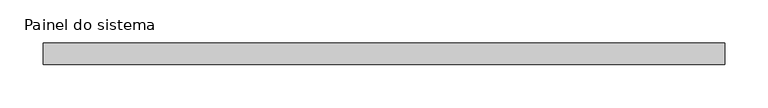
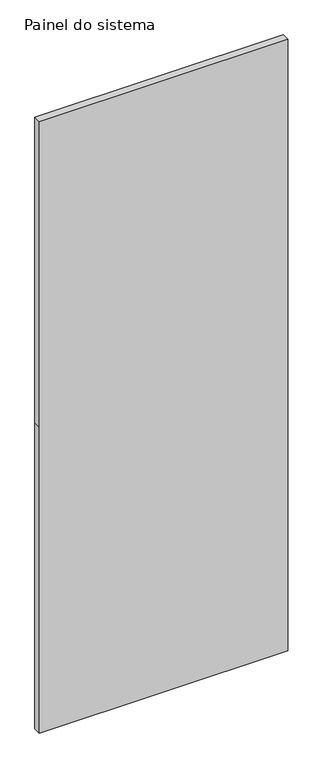
"""IFC4 building model written with IfcOpenShell, lengths in millimetres: plate geometry, Painel do sistema : Envidraçado."""

from ifc_helpers import new_model, si_unit, frame, origin, place, context, project, spatial, polyline, outline, extrude, source, transform, mapped, element, save


def painel_do_sistema_74acd235(model_context):
    return source(origin(), model_context, "Body", "SweptSolid", [
        extrude(outline(polyline([(0.0, -393.7749999), (0.0, 393.7749999), (1025.0, 393.7749999), (2050.0, 393.7749999), (2050.0, -393.7749999), (1025.0, -393.7749999), (0.0, -393.7749999)])), frame((0.0, -49.5, 0.0), z_axis=(0.0, 1.0, 0.0), x_axis=(0.0, 0.0, 1.0)), (0.0, 0.0, 1.0), 25.0),
    ])


if __name__ == "__main__":
    model = new_model("IFC4")
    model_context = context("Model", 3, world=origin())
    ifc_project = project(units=[si_unit("LENGTHUNIT", "METRE", prefix="MILLI")], contexts=[model_context])
    site = spatial("IfcSite", under=ifc_project)
    building = spatial("IfcBuilding", under=site)
    placement = place(None, origin())
    painel_do_sistema_shape = painel_do_sistema_74acd235(model_context)
    element("IfcPlate", 1, ObjectType="Painel do sistema : Envidraçado", at=placement, inside=building, context=model_context, shape_type="MappedRepresentation", body=[
        mapped(painel_do_sistema_shape, transform((0.0, 0.0, 0.0), x_axis=(1.0, 0.0, 0.0), y_axis=(0.0, 1.0, 0.0), z_axis=(0.0, 0.0, 1.0))),
    ])
    save(model, "model.ifc")

# Revit data of these elements
# Type "Painel do sistema : Envidraçado"
#   Construction Type Id = "GSP4R"
#   Analytic Construction = "Vidraça única Pilkington 1/8 pol"
#   Visual Light Transmittance = 0.9
#   Solar Heat Gain Coefficient = 0.86
#   Heat Transfer Coefficient (U) = 6.7069 W/(m²·K)
# Element 1 (IfcPlate, "Painel do sistema : Envidraçado")
#   Materials on its faces: ".VIDRO GENÉRICO"
# Materials
#   ".VIDRO GENÉRICO": class ".CC_VIDRO", colour RGB 0 128 192, transparency 0.9, Description = "Vidro comum", Cost = 0
